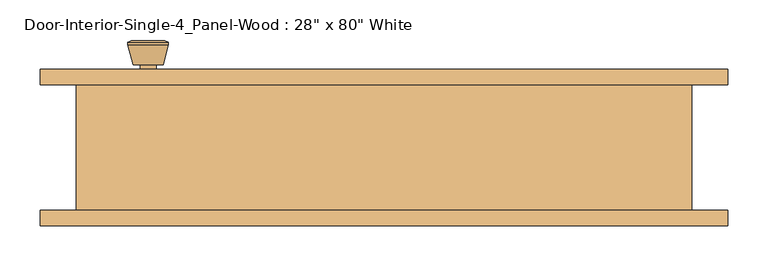
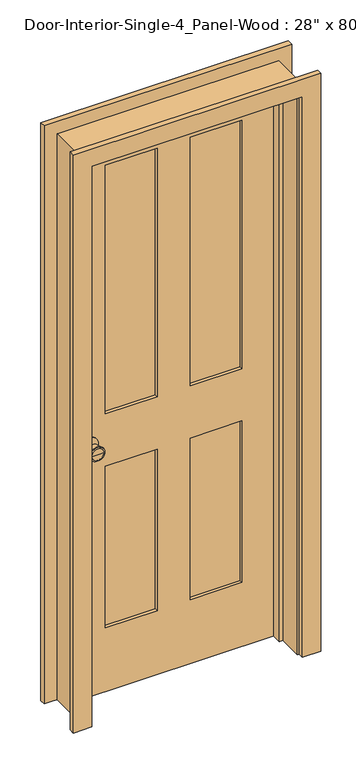
"""IFC4 building model written with IfcOpenShell, lengths in millimetres: door geometry."""

from ifc_helpers import new_model, si_unit, point, frame, frame_2d, origin, place, context, project, spatial, polyline, circle_curve, trimmed, segment, composite_curve, outline, extrude, faceted_brep, source, transform, mapped, element, save
from ifc_brep_helpers import plane_surface, cylinder_surface, revolved_surface, advanced_brep


def door_a37810f2(model_context):
    return source(origin(), model_context, "Body", "SolidModel", [
        advanced_brep(
        [(-292.1, 33.6875, 914.4), (-282.1, 33.6875, 914.4), (-302.1, 33.6875, 914.4), (-271.6241324, -15.3125, 914.4), (-292.1, -15.3125, 914.4), (-312.5758676, -15.3125, 914.4), (-267.1, -13.4846319, 914.4), (-317.1, -13.4846319, 914.4), (-267.1, -10.0209537, 914.4), (-317.1, -10.0209537, 914.4), (-273.463764, 14.6875, 914.4), (-310.736236, 14.6875, 914.4), (-282.1, 14.6875, 914.4), (-302.1, 14.6875, 914.4)],
        [
            (0, 1),
            (1, 2, circle_curve(frame((-292.1, 33.6875, 914.4), z_axis=(0.0, 1.0, 0.0), x_axis=(-1.0, 0.0, 0.0)), 10.0)),
            (2, 0),
            (2, 1, circle_curve(frame((-292.1, 33.6875, 914.4), z_axis=(0.0, 1.0, 0.0), x_axis=(-1.0, 0.0, 0.0)), 10.0)),
            (3, 4),
            (4, 5),
            (5, 3, circle_curve(frame((-292.1, -15.3125, 914.4), z_axis=(0.0, -1.0, 0.0), x_axis=(-1.0, 0.0, 0.0)), 20.4758676)),
            (3, 5, circle_curve(frame((-292.1, -15.3125, 914.4), z_axis=(0.0, -1.0, 0.0), x_axis=(-1.0, 0.0, 0.0)), 20.4758676)),
            (6, 3),
            (5, 7),
            (7, 6, circle_curve(frame((-292.1, -13.4846319, 914.4), z_axis=(0.0, -1.0, 0.0), x_axis=(-1.0, 0.0, 0.0)), 25.0)),
            (6, 7, circle_curve(frame((-292.1, -13.4846319, 914.4), z_axis=(0.0, -1.0, 0.0), x_axis=(-1.0, 0.0, 0.0)), 25.0)),
            (8, 6),
            (7, 9),
            (9, 8, circle_curve(frame((-292.1, -10.0209537, 914.4), z_axis=(0.0, -1.0, 0.0), x_axis=(-1.0, 0.0, 0.0)), 25.0)),
            (8, 9, circle_curve(frame((-292.1, -10.0209537, 914.4), z_axis=(0.0, -1.0, 0.0), x_axis=(-1.0, 0.0, 0.0)), 25.0)),
            (10, 8),
            (9, 11),
            (11, 10, circle_curve(frame((-292.1, 14.6875, 914.4), z_axis=(0.0, -1.0, 0.0), x_axis=(-1.0, 0.0, 0.0)), 18.636236)),
            (10, 11, circle_curve(frame((-292.1, 14.6875, 914.4), z_axis=(0.0, -1.0, 0.0), x_axis=(-1.0, 0.0, 0.0)), 18.636236)),
            (12, 10),
            (11, 13),
            (13, 12, circle_curve(frame((-292.1, 14.6875, 914.4), z_axis=(0.0, -1.0, 0.0), x_axis=(-1.0, 0.0, 0.0)), 10.0)),
            (12, 13, circle_curve(frame((-292.1, 14.6875, 914.4), z_axis=(0.0, -1.0, 0.0), x_axis=(-1.0, 0.0, 0.0)), 10.0)),
            (1, 12),
            (13, 2),
        ],
        [
            plane_surface(frame((-292.1, 33.6875, 914.4), z_axis=(0.0, 1.0, 0.0), x_axis=(-1.0, 0.0, 0.0))),
            plane_surface(frame((-292.1, -15.3125, 914.4), z_axis=(0.0, -1.0, 0.0), x_axis=(-1.0, 0.0, 0.0))),
            revolved_surface(polyline([(-312.5758676, -15.3125, 914.4), (-317.1, -13.4846319, 914.4)]), (-292.1, 33.6875, 914.4), (0.0, 1.0, 0.0)),
            cylinder_surface(frame((-292.1, 33.6875, 914.4), z_axis=(0.0, 1.0, 0.0), x_axis=(-1.0, 0.0, 0.0)), 25.0),
            revolved_surface(polyline([(-317.1, -10.0209537, 914.4), (-310.736236, 14.6875, 914.4)]), (-292.1, 33.6875, 914.4), (0.0, 1.0, 0.0)),
            plane_surface(frame((-292.1, 14.6875, 914.4), z_axis=(0.0, 1.0, 0.0), x_axis=(-1.0, 0.0, 0.0))),
            cylinder_surface(frame((-292.1, 33.6875, 914.4), z_axis=(0.0, 1.0, 0.0), x_axis=(-1.0, 0.0, 0.0)), 10.0),
        ],
        [
            (0, [[1, 2, 3]]),
            (0, [[-3, 4, -1]]),
            (1, [[5, 6, 7]]),
            (1, [[-6, -5, 8]]),
            (2, [[9, -7, 10, 11]]),
            (2, [[-10, -8, -9, 12]]),
            (3, [[13, -11, 14, 15]]),
            (3, [[-14, -12, -13, 16]]),
            (4, [[17, -15, 18, 19]]),
            (4, [[-18, -16, -17, 20]]),
            (5, [[21, -19, 22, 23]]),
            (5, [[-22, -20, -21, 24]]),
            (6, [[25, -23, 26, -2]]),
            (6, [[-26, -24, -25, -4]]),
        ],
    ),
        extrude(outline(composite_curve([segment(trimmed(circle_curve(frame_2d((914.4, -292.1)), 30.0), [point((914.4, -322.1))], [point((914.4, -262.1))], False, "CARTESIAN"), True, "CONTINUOUS"), segment(trimmed(circle_curve(frame_2d((914.4, -292.1)), 30.0), [point((914.4, -262.1))], [point((914.4, -322.1))], False, "CARTESIAN"), True, "CONTINUOUS")], self_intersect=False)), frame((0.0, 33.6875, 0.0), z_axis=(0.0, 1.0, 0.0), x_axis=(0.0, 0.0, 1.0)), (0.0, 0.0, 1.0), 6.0),
        advanced_brep(
        [(-292.1, 80.6125, 914.4), (-302.1, 80.6125, 914.4), (-282.1, 80.6125, 914.4), (-271.6241324, 129.6125, 914.4), (-312.5758676, 129.6125, 914.4), (-292.1, 129.6125, 914.4), (-267.1, 127.7846319, 914.4), (-317.1, 127.7846319, 914.4), (-267.1, 124.3209537, 914.4), (-317.1, 124.3209537, 914.4), (-273.463764, 99.6125, 914.4), (-310.736236, 99.6125, 914.4), (-282.1, 99.6125, 914.4), (-302.1, 99.6125, 914.4)],
        [
            (0, 1),
            (1, 2, circle_curve(frame((-292.1, 80.6125, 914.4), z_axis=(0.0, -1.0, 0.0), x_axis=(-1.0, 0.0, 0.0)), 10.0)),
            (2, 0),
            (2, 1, circle_curve(frame((-292.1, 80.6125, 914.4), z_axis=(0.0, -1.0, 0.0), x_axis=(-1.0, 0.0, 0.0)), 10.0)),
            (3, 4, circle_curve(frame((-292.1, 129.6125, 914.4), z_axis=(0.0, 1.0, 0.0), x_axis=(-1.0, 0.0, 0.0)), 20.4758676)),
            (4, 5),
            (5, 3),
            (4, 3, circle_curve(frame((-292.1, 129.6125, 914.4), z_axis=(0.0, 1.0, 0.0), x_axis=(-1.0, 0.0, 0.0)), 20.4758676)),
            (6, 7, circle_curve(frame((-292.1, 127.7846319, 914.4), z_axis=(0.0, 1.0, 0.0), x_axis=(-1.0, 0.0, 0.0)), 25.0)),
            (7, 4),
            (3, 6),
            (7, 6, circle_curve(frame((-292.1, 127.7846319, 914.4), z_axis=(0.0, 1.0, 0.0), x_axis=(-1.0, 0.0, 0.0)), 25.0)),
            (8, 9, circle_curve(frame((-292.1, 124.3209537, 914.4), z_axis=(0.0, 1.0, 0.0), x_axis=(-1.0, 0.0, 0.0)), 25.0)),
            (9, 7),
            (6, 8),
            (9, 8, circle_curve(frame((-292.1, 124.3209537, 914.4), z_axis=(0.0, 1.0, 0.0), x_axis=(-1.0, 0.0, 0.0)), 25.0)),
            (10, 11, circle_curve(frame((-292.1, 99.6125, 914.4), z_axis=(0.0, 1.0, 0.0), x_axis=(-1.0, 0.0, 0.0)), 18.636236)),
            (11, 9),
            (8, 10),
            (11, 10, circle_curve(frame((-292.1, 99.6125, 914.4), z_axis=(0.0, 1.0, 0.0), x_axis=(-1.0, 0.0, 0.0)), 18.636236)),
            (12, 13, circle_curve(frame((-292.1, 99.6125, 914.4), z_axis=(0.0, 1.0, 0.0), x_axis=(-1.0, 0.0, 0.0)), 10.0)),
            (13, 11),
            (10, 12),
            (13, 12, circle_curve(frame((-292.1, 99.6125, 914.4), z_axis=(0.0, 1.0, 0.0), x_axis=(-1.0, 0.0, 0.0)), 10.0)),
            (1, 13),
            (12, 2),
        ],
        [
            plane_surface(frame((-292.1, 80.6125, 914.4), z_axis=(0.0, -1.0, 0.0), x_axis=(-1.0, 0.0, 0.0))),
            plane_surface(frame((-292.1, 129.6125, 914.4), z_axis=(0.0, 1.0, 0.0), x_axis=(-1.0, 0.0, 0.0))),
            revolved_surface(polyline([(-312.5758676, 129.6125, 914.4), (-317.1, 127.7846319, 914.4)]), (-292.1, 80.6125, 914.4), (0.0, -1.0, 0.0)),
            cylinder_surface(frame((-292.1, 80.6125, 914.4), z_axis=(0.0, -1.0, 0.0), x_axis=(-1.0, 0.0, 0.0)), 25.0),
            revolved_surface(polyline([(-317.1, 124.3209537, 914.4), (-310.736236, 99.6125, 914.4)]), (-292.1, 80.6125, 914.4), (0.0, -1.0, 0.0)),
            plane_surface(frame((-292.1, 99.6125, 914.4), z_axis=(0.0, -1.0, 0.0), x_axis=(-1.0, 0.0, 0.0))),
            cylinder_surface(frame((-292.1, 80.6125, 914.4), z_axis=(0.0, -1.0, 0.0), x_axis=(-1.0, 0.0, 0.0)), 10.0),
        ],
        [
            (0, [[1, 2, 3]]),
            (0, [[-3, 4, -1]]),
            (1, [[5, 6, 7]]),
            (1, [[8, -7, -6]]),
            (2, [[9, 10, -5, 11]]),
            (2, [[12, -11, -8, -10]]),
            (3, [[13, 14, -9, 15]]),
            (3, [[16, -15, -12, -14]]),
            (4, [[17, 18, -13, 19]]),
            (4, [[20, -19, -16, -18]]),
            (5, [[21, 22, -17, 23]]),
            (5, [[24, -23, -20, -22]]),
            (6, [[-2, 25, -21, 26]]),
            (6, [[-4, -26, -24, -25]]),
        ],
    ),
        extrude(outline(composite_curve([segment(trimmed(circle_curve(frame_2d((914.4, -292.1)), 30.0), [point((914.4, -322.1))], [point((914.4, -262.1))], False, "CARTESIAN"), True, "CONTINUOUS"), segment(trimmed(circle_curve(frame_2d((914.4, -292.1)), 30.0), [point((914.4, -262.1))], [point((914.4, -322.1))], False, "CARTESIAN"), True, "CONTINUOUS")], self_intersect=False)), frame((0.0, 74.6125, 0.0), z_axis=(0.0, 1.0, 0.0), x_axis=(0.0, 0.0, 1.0)), (0.0, 0.0, 1.0), 6.0),
        extrude(outline(polyline([(234.95, 51.3291667), (57.15, 51.3291667), (57.15, 62.9708333), (234.95, 62.9708333), (234.95, 51.3291667)])), frame((0.0, 0.0, 1009.65), z_axis=(0.0, 0.0, 1.0), x_axis=(1.0, 0.0, 0.0)), (0.0, 0.0, 1.0), 903.2875),
        extrude(outline(polyline([(-57.15, 51.3291667), (-234.95, 51.3291667), (-234.95, 62.9708333), (-57.15, 62.9708333), (-57.15, 51.3291667)])), frame((0.0, 0.0, 1009.65), z_axis=(0.0, 0.0, 1.0), x_axis=(1.0, 0.0, 0.0)), (0.0, 0.0, 1.0), 903.2875),
        extrude(outline(polyline([(234.95, 51.3291667), (57.15, 51.3291667), (57.15, 62.9708333), (234.95, 62.9708333), (234.95, 51.3291667)])), frame((0.0, 0.0, 231.775), z_axis=(0.0, 0.0, 1.0), x_axis=(1.0, 0.0, 0.0)), (0.0, 0.0, 1.0), 587.375),
        extrude(outline(polyline([(-57.15, 51.3291667), (-234.95, 51.3291667), (-234.95, 62.9708333), (-57.15, 62.9708333), (-57.15, 51.3291667)])), frame((0.0, 0.0, 231.775), z_axis=(0.0, 0.0, 1.0), x_axis=(1.0, 0.0, 0.0)), (0.0, 0.0, 1.0), 587.375),
        extrude(outline(polyline([(2032.0, -355.6), (0.0, -355.6), (0.0, 355.6), (2032.0, 355.6), (2032.0, -355.6)]), holes=[polyline([(1912.9375, 57.15), (1912.9375, 234.95), (1009.65, 234.95), (1009.65, 57.15), (1912.9375, 57.15)]), polyline([(1009.65, -57.15), (1009.65, -234.95), (1912.9375, -234.95), (1912.9375, -57.15), (1009.65, -57.15)]), polyline([(819.15, 57.15), (819.15, 234.95), (231.775, 234.95), (231.775, 57.15), (819.15, 57.15)]), polyline([(231.775, -57.15), (231.775, -234.95), (819.15, -234.95), (819.15, -57.15), (231.775, -57.15)])]), frame((0.0, 39.6875, 0.0), z_axis=(0.0, 1.0, 0.0), x_axis=(0.0, 0.0, 1.0)), (0.0, 0.0, 1.0), 34.925),
        faceted_brep([(381.0, 74.6125, 0.0), (381.0, -80.9625, 0.0), (355.6, -80.9625, 0.0), (355.6, 4.7625, 0.0), (342.9, 4.7625, 0.0), (342.9, 39.6875, 0.0), (355.6, 39.6875, 0.0), (355.6, 74.6125, 0.0), (381.0, 74.6125, 2057.4), (381.0, -80.9625, 2057.4), (-381.0, -80.9625, 2057.4), (-381.0, -80.9625, 0.0), (-355.6, -80.9625, 0.0), (-355.6, -80.9625, 2032.0), (355.6, -80.9625, 2032.0), (355.6, 4.7625, 2032.0), (-355.6, 4.7625, 2032.0), (-355.6, 4.7625, 0.0), (-342.9, 4.7625, 0.0), (-342.9, 4.7625, 2019.3), (342.9, 4.7625, 2019.3), (342.9, 39.6875, 2019.3), (-342.9, 39.6875, 2019.3), (-342.9, 39.6875, 0.0), (-355.6, 39.6875, 0.0), (-355.6, 39.6875, 2032.0), (355.6, 39.6875, 2032.0), (355.6, 74.6125, 2032.0), (-355.6, 74.6125, 2032.0), (-355.6, 74.6125, 0.0), (-381.0, 74.6125, 0.0), (-381.0, 74.6125, 2057.4)], [[[0, 1, 2, 3, 4, 5, 6, 7]], [[1, 0, 8, 9]], [[2, 1, 9, 10, 11, 12, 13, 14]], [[3, 2, 14, 15]], [[4, 3, 15, 16, 17, 18, 19, 20]], [[5, 4, 20, 21]], [[6, 5, 21, 22, 23, 24, 25, 26]], [[7, 6, 26, 27]], [[0, 7, 27, 28, 29, 30, 31, 8]], [[9, 8, 31, 10]], [[15, 14, 13, 16]], [[21, 20, 19, 22]], [[27, 26, 25, 28]], [[30, 29, 24, 23, 18, 17, 12, 11]], [[10, 31, 30, 11]], [[16, 13, 12, 17]], [[22, 19, 18, 23]], [[28, 25, 24, 29]]]),
        extrude(outline(polyline([(0.0, 361.95), (0.0, 425.45), (2101.85, 425.45), (2101.85, -425.45), (0.0, -425.45), (0.0, -361.95), (2038.35, -361.95), (2038.35, 361.95), (0.0, 361.95)])), frame((0.0, -100.0125, 0.0), z_axis=(0.0, 1.0, 0.0), x_axis=(0.0, 0.0, 1.0)), (0.0, 0.0, 1.0), 19.05),
        extrude(outline(polyline([(0.0, 361.95), (0.0, 425.45), (2101.85, 425.45), (2101.85, -425.45), (0.0, -425.45), (0.0, -361.95), (2038.35, -361.95), (2038.35, 361.95), (0.0, 361.95)])), frame((0.0, 74.6125, 0.0), z_axis=(0.0, 1.0, 0.0), x_axis=(0.0, 0.0, 1.0)), (0.0, 0.0, 1.0), 19.05),
    ])


if __name__ == "__main__":
    model = new_model("IFC4")
    model_context = context("Model", 3, world=origin())
    ifc_project = project(units=[si_unit("LENGTHUNIT", "METRE", prefix="MILLI")], contexts=[model_context])
    site = spatial("IfcSite", under=ifc_project)
    building = spatial("IfcBuilding", under=site)
    placement = place(None, origin())
    door_shape = door_a37810f2(model_context)
    element("IfcDoor", 1, ObjectType="Door-Interior-Single-4_Panel-Wood : 28\" x 80\" White", at=placement, inside=building, context=model_context, shape_type="MappedRepresentation", body=[
        mapped(door_shape, transform((0.0, 0.0, 0.0), x_axis=(1.0, 0.0, 0.0), y_axis=(0.0, 1.0, 0.0), z_axis=(0.0, 0.0, 1.0))),
    ])
    save(model, "model.ifc")

# Revit data of these elements
# Type "Door-Interior-Single-4_Panel-Wood : 28\" x 80\" White"
#   Type Mark = "72"
#   COBie.Type.CreatedBy = "doug.wood@us.ibm.com"
#   COBie.Type.CreatedOn = "2016-04-14T02:07:24"
#   COBie.Type.Name = "Doors_Door-Interior-Single-4_Panel-Wood_28\" x 80\" White_72"
#   COBie.Type.Category = "23-30 10 00 : Doors"
#   COBie.Type.Description = "Door-Interior-Single-4_Panel-Wood_28\" x 80\" White"
#   COBie.Type.Manufacturer = ""
#   COBie.Type.ModelNumber = ""
#   Assembly Code = "C1020300"
#   Analytic Construction = "Wooden"
#   COBie.Type.ReplacementCost = 0
#   Top Rail = 0' - 4 11/16"
#   Thickness = 0' - 1 3/8"
#   Thermal Resistance (R) = 0.455703 (m²·K)/W
#   Swing Angle [instance default] = 90.00°
#   Stiles = 0' - 4 3/4"
#   Rough Width = 2' - 6"
#   Rough Height = 6' - 9"
#   Mullion = 0' - 4 1/2"
#   Lock Rail = 0' - 7 1/2"
#   Height = 6' - 8"
#   Width = 2' - 4"
#   Heat Transfer Coefficient (U) = 2.19465 W/(m²·K)
#   Bottom Rail = 0' - 9 1/8"
#   COBie.Type = no
#   Trim Material = Trim - White
#   Panel Material = Door - Panel - White
#   Frame Material = Door - Panel - White
#   Door Handle Material = ARCAT - Metal - Brass, Polished
#   Visual Light Transmittance = 0
#   Solar Heat Gain Coefficient = 0
#   Wall Closure = (empty or 0)
#   Function = (empty or 0)
# Element 1 (IfcDoor, "Door-Interior-Single-4_Panel-Wood : 28\" x 80\" White")
#   Materials on its faces: "Door - Panel - White", "ARCAT - Metal - Brass, Polished", "Trim - White"
# Materials
#   "Trim - White": class "Wood", colour RGB 255 255 255, transparency 0, Cost = 0
#   "Door - Panel - White": class "Wood", colour RGB 255 255 255, transparency 0, Cost = 0
#   "ARCAT - Metal - Brass, Polished": class "Unassigned", colour RGB 246 240 166, transparency 0, Keynote = "05050", Model = "Generic", Manufacturer = "Generic", Description = "Steel, Chrome Plated"
